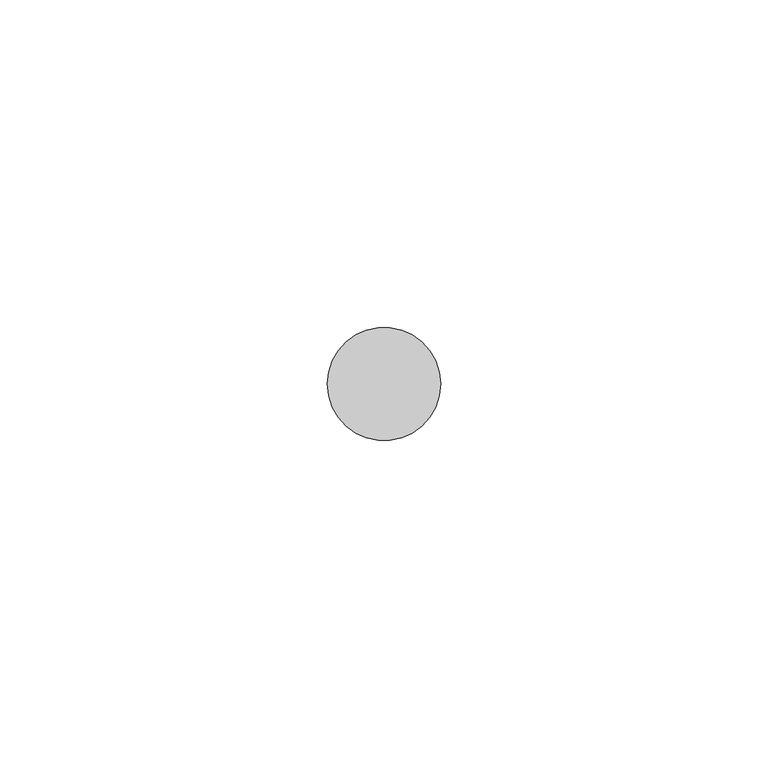
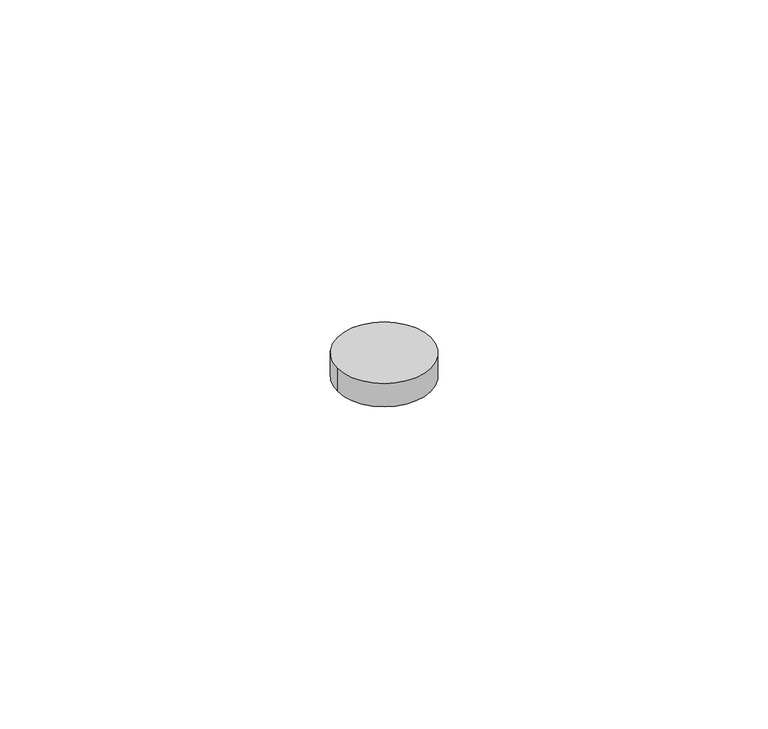
"""IFC4 building model written with IfcOpenShell, lengths in millimetres: proxy geometry, Hinge Pin Keeper1 : Hinge Pin Keeper."""

from ifc_helpers import new_model, si_unit, point, frame, frame_2d, origin, place, context, project, spatial, circle_curve, trimmed, segment, composite_curve, outline, extrude, source, transform, mapped, element, save


def generic_models_13552f7c(model_context):
    return source(origin(), model_context, "Body", "SweptSolid", [
        extrude(outline(composite_curve([segment(trimmed(circle_curve(frame_2d((587319.1320739, -531776.6049841)), 8.6534625), [point((587310.4786114, -531776.6049841))], [point((587327.7855364, -531776.6049841))], False, "CARTESIAN"), True, "CONTINUOUS"), segment(trimmed(circle_curve(frame_2d((587319.1320739, -531776.6049841)), 8.6534625), [point((587327.7855364, -531776.6049841))], [point((587310.4786114, -531776.6049841))], False, "CARTESIAN"), True, "CONTINUOUS")], self_intersect=False)), frame((0.0, 0.0, 2084.5859375), z_axis=(0.0, 0.0, 1.0), x_axis=(1.0, 0.0, 0.0)), (0.0, 0.0, 1.0), 4.5640625),
    ])


if __name__ == "__main__":
    model = new_model("IFC4")
    model_context = context("Model", 3, world=origin())
    ifc_project = project(units=[si_unit("LENGTHUNIT", "METRE", prefix="MILLI")], contexts=[model_context])
    site = spatial("IfcSite", under=ifc_project)
    building = spatial("IfcBuilding", under=site)
    placement = place(None, origin())
    generic_models_shape = generic_models_13552f7c(model_context)
    element("IfcBuildingElementProxy", 1, Name="Hinge Pin Keeper1 : Hinge Pin Keeper", ObjectType="Hinge Pin Keeper1 : Hinge Pin Keeper", at=placement, inside=building, context=model_context, shape_type="MappedRepresentation", body=[
        mapped(generic_models_shape, transform((0.0, 0.0, 0.0), x_axis=(1.0, 0.0, 0.0), y_axis=(0.0, 1.0, 0.0), z_axis=(0.0, 0.0, 1.0))),
    ])
    save(model, "model.ifc")

# Revit data of these elements
# Element 1 (IfcBuildingElementProxy, "Hinge Pin Keeper1 : Hinge Pin Keeper")
#   Materials on its faces: "6\"X6\" WELD-ON STL BUTT HINGE"
# Materials
#   "6\"X6\" WELD-ON STL BUTT HINGE": class "Metal", colour RGB 189 187 185, transparency 0, Description = "Carbon steel", Cost = 0
